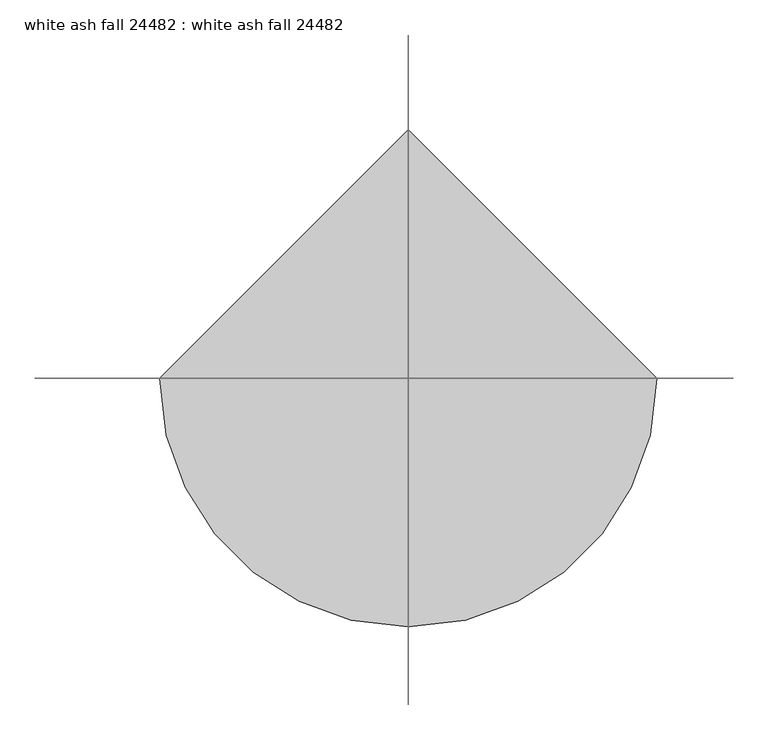
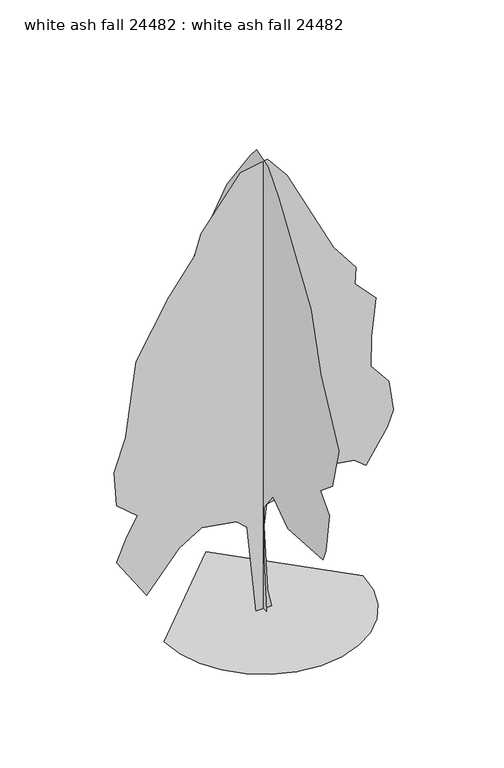
"""IFC4 building model written with IfcOpenShell, lengths in millimetres: proxy geometry, white ash fall 24482 : white ash fall 24482."""

from ifc_helpers import new_model, si_unit, origin, place, context, project, spatial, triangles, source, transform, mapped, element, save


def white_ash_fall_24482_white_ash_fall_24482_ca342e74(model_context):
    return source(origin(), model_context, "Body", "Tessellation", [
        triangles([(-1903.1117432, 0.0, 0.0), (-1852.7994072, -436.0675326, 0.0), (-1709.5128044, -836.5267736, 0.0), (-1484.7201302, -1189.902079, 0.0), (-1189.902079, -1484.7201302, 0.0), (-836.5243029, -1709.5103336, 0.0), (-436.0675326, -1852.7994072, 0.0), (8.32e-05, -1903.1117432, 0.0), (436.0675326, -1852.7994072, 0.0), (836.5267736, -1709.5128044, 0.0), (1189.902079, -1484.7201302, 0.0), (1484.7201302, -1189.902079, 0.0), (1709.5103336, -836.5243029, 0.0), (1852.7994072, -436.0675326, 0.0), (1903.1117432, 0.0001664, 0.0), (-0.0002496, 1903.1117432, 0.0), (-6.4e-06, -107.924944, 0.0613456), (2.91e-05, -19.1547901, 1015.9932175), (6.03e-05, -22.4623803, 2068.4709812), (5.39e-05, -325.6028727, 2458.2394867), (1.45e-05, -807.5987429, 2100.6274487), (-5.27e-05, -1977.9757782, 2188.0796688), (-5.09e-05, -2067.0104599, 2427.1421116), (-3.51e-05, -2191.3969082, 3204.5680595), (-7.8e-06, -1895.979475, 3531.0600494), (-2.12e-05, -2284.6861267, 3857.5773285), (-9.2e-06, -2502.3617935, 4697.2004974), (6.13e-05, -1911.529398, 5878.860347), (0.0001153, -1572.9038464, 7015.6124725), (0.0002258, -512.181237, 8599.811705), (0.0002601, -154.5713246, 9035.1682709), (0.0002865, 234.1363626, 9144.0075577), (0.0002913, 433.9238045, 8906.4918228), (0.0003064, 1213.6790434, 7853.5084213), (0.0003087, 2239.8677868, 5877.6918137), (0.0003058, 2576.679641, 5106.6993393), (0.0002851, 2628.5718224, 4308.4785851), (0.0002675, 2473.0932312, 4028.6209579), (0.000235, 2395.3514648, 3095.7290634), (0.0002321, 2555.4707611, 2675.9174789), (0.0001966, 2115.4813385, 2364.9501228), (0.0001827, 2177.675798, 1774.1152565), (0.0001544, 1919.8426987, 1341.3319347), (0.0001354, 1726.7746868, 1089.9885555), (9.37e-05, 700.5858707, 1743.0180267), (9e-05, 514.0075064, 1991.7909233), (7.64e-05, 345.4377448, 1871.6004398), (4.67e-05, 163.0671178, 1239.2314808), (5.8e-06, 97.9767685, 0.0613703), (-139.7232302, 6.1e-06, 0.0682885), (-310.5051023, -0.0001955, 1753.6784225), (-510.5150233, -0.0002089, 1939.8629883), (-1184.5807468, -0.0001927, 2050.8713287), (-1618.5299858, -0.0001419, 1783.914513), (-2238.7425648, -2.84e-05, 1058.8988834), (-2814.0427689, -0.0001052, 1914.0565693), (-2611.9094673, -0.0001696, 2380.5051327), (-2409.7761658, -0.0002192, 2722.5774216), (-2814.0427689, -0.0002423, 3064.6393913), (-2860.6774223, -0.0003218, 3748.7636215), (-2642.9991394, -0.0004074, 4386.2279091), (-2440.8707794, -0.0005904, 5847.7703842), (-1817.4934227, -0.0007464, 6927.6777237), (-1321.3953609, -0.0008469, 7589.1960663), (-1197.0064419, -0.0009024, 8008.9820709), (-435.1404453, -0.0010506, 8972.9889267), (77.9529181, -0.0010842, 9066.2832321), (451.1119632, -0.0010468, 8615.3822662), (1343.785564, -0.0008745, 6842.8672028), (1771.7911251, -0.0008273, 6290.4422012), (1757.1683258, -0.0007869, 5956.609671), (2157.6860298, -0.0007547, 5539.8967346), (2072.4358555, -0.0006605, 4780.5631416), (2056.3779694, -0.0005886, 4183.7135262), (2399.5679226, -0.0005536, 3764.3083122), (2487.9397087, -0.0004852, 3157.9084076), (2379.1005672, -0.0004434, 2846.9613991), (1961.5166084, -0.0003491, 2209.4741478), (1741.621019, -0.0003618, 2396.0524395), (1104.141398, -0.0003453, 2491.7598244), (637.6903639, -0.0003117, 2380.5051327), (353.060281, -0.0002734, 2163.9953831), (54.4347815, -0.000252, 2094.0056145), (14.3638898, -0.0002002, 1674.2703335), (82.551847, -4.67e-05, 361.775047), (152.5283897, -6.7e-06, 0.0682758)], [[15, 16, 1], [14, 15, 1], [14, 1, 2], [13, 14, 2], [13, 2, 3], [13, 3, 4], [12, 13, 4], [11, 12, 4], [11, 4, 5], [11, 5, 6], [11, 6, 7], [11, 7, 8], [11, 8, 9], [11, 9, 10], [48, 49, 17], [48, 17, 18], [48, 18, 19], [47, 48, 19], [43, 44, 45], [42, 43, 45], [41, 42, 45], [41, 45, 46], [39, 40, 41], [31, 32, 33], [21, 22, 23], [21, 23, 24], [21, 24, 25], [20, 21, 25], [46, 47, 19], [30, 31, 33], [30, 33, 34], [29, 30, 34], [29, 34, 35], [28, 29, 35], [28, 35, 36], [28, 36, 37], [28, 37, 38], [27, 28, 38], [26, 27, 38], [25, 26, 38], [20, 25, 38], [20, 38, 39], [20, 39, 41], [20, 41, 46], [20, 46, 19], [85, 86, 50], [85, 50, 51], [84, 85, 51], [54, 55, 56], [54, 56, 57], [77, 78, 79], [83, 84, 51], [83, 51, 52], [54, 57, 58], [53, 54, 58], [66, 67, 68], [65, 66, 68], [65, 68, 69], [64, 65, 69], [63, 64, 69], [62, 63, 69], [61, 62, 69], [61, 69, 70], [61, 70, 71], [61, 71, 72], [61, 72, 73], [61, 73, 74], [60, 61, 74], [59, 60, 74], [58, 59, 74], [53, 58, 74], [52, 53, 74], [83, 52, 74], [82, 83, 74], [81, 82, 74], [80, 81, 74], [80, 74, 75], [79, 80, 75], [77, 79, 75], [77, 75, 76]], closed=False),
    ])


if __name__ == "__main__":
    model = new_model("IFC4")
    model_context = context("Model", 3, world=origin())
    ifc_project = project(units=[si_unit("LENGTHUNIT", "METRE", prefix="MILLI")], contexts=[model_context])
    site = spatial("IfcSite", under=ifc_project)
    building = spatial("IfcBuilding", under=site)
    placement = place(None, origin())
    white_ash_fall_24482_white_ash_fall_24482_shape = white_ash_fall_24482_white_ash_fall_24482_ca342e74(model_context)
    element("IfcBuildingElementProxy", 1, Name="white ash fall 24482 : white ash fall 24482", ObjectType="white ash fall 24482 : white ash fall 24482", at=placement, inside=building, context=model_context, shape_type="MappedRepresentation", body=[
        mapped(white_ash_fall_24482_white_ash_fall_24482_shape, transform((0.0, 0.0, 0.0), x_axis=(1.0, 0.0, 0.0), y_axis=(0.0, 1.0, 0.0), z_axis=(0.0, 0.0, 1.0))),
    ])
    save(model, "model.ifc")

# Revit data of these elements
# Type "white ash fall 24482 : white ash fall 24482"
#   built-in parameter 1005195 = "RPC-16-G1AF-G8PX-CFC7-2000-ST1L-LVER-AU"
#   Height = 0
